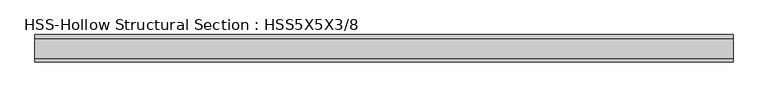
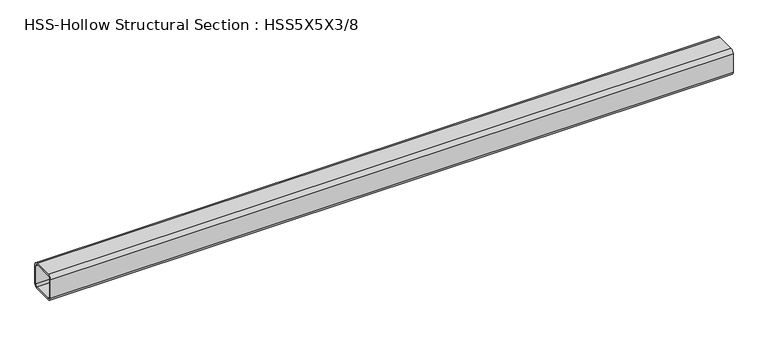
"""IFC4 building model written with IfcOpenShell, lengths in millimetres: member geometry, HSS-Hollow Structural Section : HSS5X5X3/8."""

from ifc_helpers import new_model, si_unit, point, frame, frame_2d, origin, place, context, project, spatial, polyline, circle_curve, trimmed, segment, composite_curve, outline, extrude, source, transform, mapped, element, save


def hss_hollow_structural_section_hss5x5x3_8_1bfc15f5(model_context):
    return source(origin(), model_context, "Body", "SweptSolid", [
        extrude(outline(composite_curve([segment(polyline([(63.5, 45.7708), (63.5, -45.7708)]), True, "CONTINUOUS"), segment(trimmed(circle_curve(frame_2d((45.7708, -45.7708)), 17.7292), [point((63.5, -45.7708))], [point((45.7708, -63.5))], False, "CARTESIAN"), True, "CONTINUOUS"), segment(polyline([(45.7708, -63.5), (-45.7708, -63.5)]), True, "CONTINUOUS"), segment(trimmed(circle_curve(frame_2d((-45.7708, -45.7708)), 17.7292), [point((-45.7708, -63.5))], [point((-63.5, -45.7708))], False, "CARTESIAN"), True, "CONTINUOUS"), segment(polyline([(-63.5, -45.7708), (-63.5, 45.7708)]), True, "CONTINUOUS"), segment(trimmed(circle_curve(frame_2d((-45.7708, 45.7708)), 17.7292), [point((-63.5, 45.7708))], [point((-45.7708, 63.5))], False, "CARTESIAN"), True, "CONTINUOUS"), segment(polyline([(-45.7708, 63.5), (45.7708, 63.5)]), True, "CONTINUOUS"), segment(trimmed(circle_curve(frame_2d((45.7708, 45.7708)), 17.7292), [point((45.7708, 63.5))], [point((63.5, 45.7708))], False, "CARTESIAN"), True, "CONTINUOUS")], self_intersect=False), holes=[composite_curve([segment(trimmed(circle_curve(frame_2d((-45.7708, 45.7708)), 8.8646), [point((-45.7708, 54.6354))], [point((-54.6354, 45.7708))], True, "CARTESIAN"), True, "CONTINUOUS"), segment(polyline([(-54.6354, 45.7708), (-54.6354, -45.7708)]), True, "CONTINUOUS"), segment(trimmed(circle_curve(frame_2d((-45.7708, -45.7708)), 8.8646), [point((-54.6354, -45.7708))], [point((-45.7708, -54.6354))], True, "CARTESIAN"), True, "CONTINUOUS"), segment(polyline([(-45.7708, -54.6354), (45.7708, -54.6354)]), True, "CONTINUOUS"), segment(trimmed(circle_curve(frame_2d((45.7708, -45.7708)), 8.8646), [point((45.7708, -54.6354))], [point((54.6354, -45.7708))], True, "CARTESIAN"), True, "CONTINUOUS"), segment(polyline([(54.6354, -45.7708), (54.6354, 45.7708)]), True, "CONTINUOUS"), segment(trimmed(circle_curve(frame_2d((45.7708, 45.7708)), 8.8646), [point((54.6354, 45.7708))], [point((45.7708, 54.6354))], True, "CARTESIAN"), True, "CONTINUOUS"), segment(polyline([(45.7708, 54.6354), (-45.7708, 54.6354)]), True, "CONTINUOUS")], self_intersect=False)]), frame((-1559.4617293, 0.0, 0.0), z_axis=(1.0, 0.0, 0.0), x_axis=(0.0, 1.0, 0.0)), (0.0, 0.0, 1.0), 3220.1428771),
    ])


if __name__ == "__main__":
    model = new_model("IFC4")
    model_context = context("Model", 3, world=origin())
    ifc_project = project(units=[si_unit("LENGTHUNIT", "METRE", prefix="MILLI")], contexts=[model_context])
    site = spatial("IfcSite", under=ifc_project)
    building = spatial("IfcBuilding", under=site)
    placement = place(None, origin())
    hss_hollow_structural_section_hss5x5x3_8_shape = hss_hollow_structural_section_hss5x5x3_8_1bfc15f5(model_context)
    element("IfcMember", 1, ObjectType="HSS-Hollow Structural Section : HSS5X5X3/8", at=placement, inside=building, context=model_context, shape_type="MappedRepresentation", body=[
        mapped(hss_hollow_structural_section_hss5x5x3_8_shape, transform((0.0, 0.0, 0.0), x_axis=(1.0, 0.0, 0.0), y_axis=(0.0, 1.0, 0.0), z_axis=(0.0, 0.0, 1.0))),
    ])
    save(model, "model.ifc")

# Revit data of these elements
# Type "HSS-Hollow Structural Section : HSS5X5X3/8"
#   Assembly Code = "B10"
#   Shape = "Square"
#   W = 22.3
#   Ht = 0' - 5"
#   Length [instance default] = 5' - 0"
#   b = 0' - 5"
#   kr = 0' - 0.698"
#   t = 0' - 0.349"
#   A = 0.0429167 SF
#   Structural Material [instance default] = Steel ASTM A500, Grade B, Rectangular and Square
# Element 1 (IfcMember, "HSS-Hollow Structural Section : HSS5X5X3/8")
#   Materials on its faces: "Steel ASTM A500, Grade B, Rectangular and Square"
# Materials
#   "Steel ASTM A500, Grade B, Rectangular and Square": class "Metal", colour RGB 199 199 199, transparency 0, Description = "Carbon steel", Cost = 0
